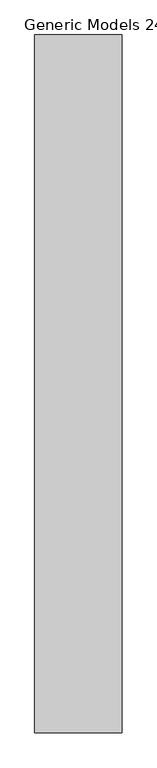
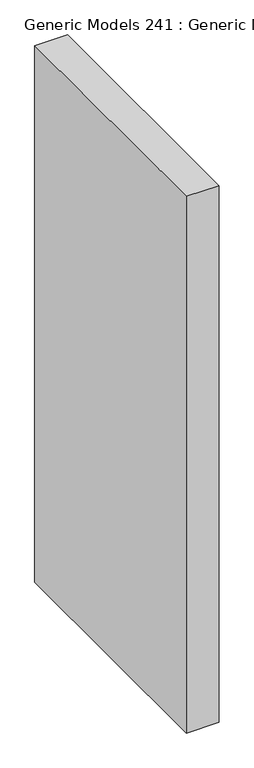
"""IFC4 building model written with IfcOpenShell, lengths in millimetres: proxy geometry, Generic Models 241 : Generic Models 1."""

from ifc_helpers import new_model, si_unit, frame, origin, place, context, project, spatial, polyline, outline, extrude, source, transform, mapped, element, save


def generic_models_241_generic_models_1_d4f8735c(model_context):
    return source(origin(), model_context, "Body", "SweptSolid", [
        extrude(outline(polyline([(48469.55, 1219.2), (48469.55, 0.0), (48317.15, 0.0), (48317.15, 1219.2), (48469.55, 1219.2)])), frame((0.0, 0.0, 3048.0), z_axis=(0.0, 0.0, 1.0), x_axis=(1.0, 0.0, 0.0)), (0.0, 0.0, 1.0), 2633.9569015),
    ])


if __name__ == "__main__":
    model = new_model("IFC4")
    model_context = context("Model", 3, world=origin())
    ifc_project = project(units=[si_unit("LENGTHUNIT", "METRE", prefix="MILLI")], contexts=[model_context])
    site = spatial("IfcSite", under=ifc_project)
    building = spatial("IfcBuilding", under=site)
    placement = place(None, origin())
    generic_models_241_generic_models_1_shape = generic_models_241_generic_models_1_d4f8735c(model_context)
    element("IfcBuildingElementProxy", 1, Name="Generic Models 241 : Generic Models 1", ObjectType="Generic Models 241 : Generic Models 1", at=placement, inside=building, context=model_context, shape_type="MappedRepresentation", body=[
        mapped(generic_models_241_generic_models_1_shape, transform((0.0, 0.0, 0.0), x_axis=(1.0, 0.0, 0.0), y_axis=(0.0, 1.0, 0.0), z_axis=(0.0, 0.0, 1.0))),
    ])
    save(model, "model.ifc")

# Revit data of these elements
# Element 1 (IfcBuildingElementProxy, "Generic Models 241 : Generic Models 1")
#   Materials on its faces: "EXISTING WALL"
# Materials
#   "EXISTING WALL": class "Generic", colour RGB 201 201 201, transparency 0, Cost = 0
